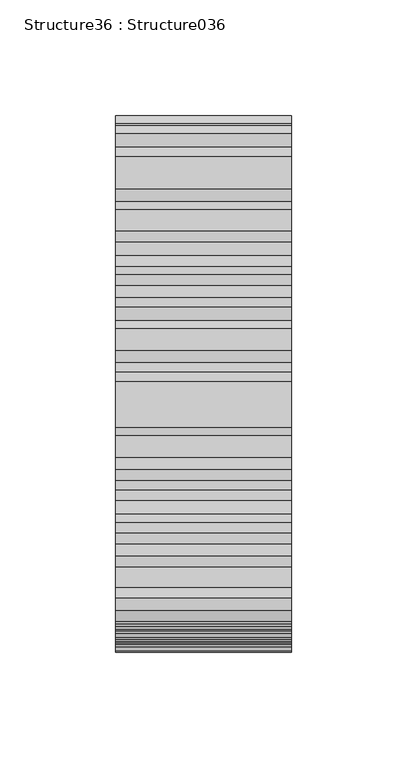
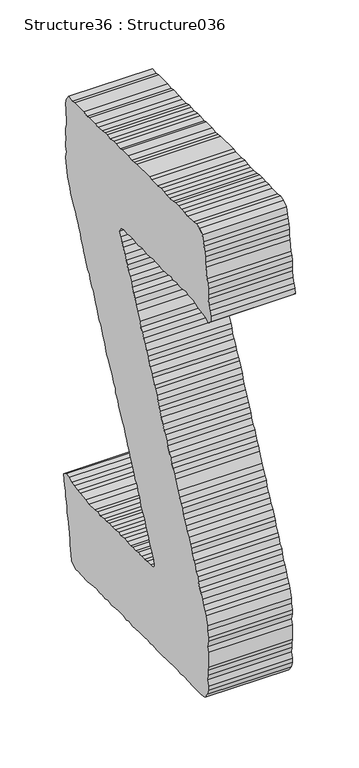
"""IFC4 building model written with IfcOpenShell, lengths in millimetres: proxy geometry, Structure36 : Structure036."""

from ifc_helpers import new_model, si_unit, frame, origin, place, context, project, spatial, polyline, outline, extrude, source, transform, mapped, element, save


def structure36_structure036_21f55036(model_context):
    return source(origin(), model_context, "Body", "SweptSolid", [
        extrude(outline(polyline([(252723.5287775, 3631.3410106), (252722.9447015, 3626.0554434), (252721.770131, 3621.3732075), (252720.5843283, 3616.69739), (252720.5843283, 3612.0135494), (252718.8353094, 3606.7295868), (252718.2512334, 3602.6298224), (252717.6607389, 3597.3538828), (252716.4845638, 3592.6700423), (252715.91172, 3589.1527492), (252714.7355449, 3584.4689087), (252714.1530735, 3579.7690221), (252713.5609744, 3573.9266571), (252713.5609744, 3569.8268927), (252712.3944269, 3565.1254015), (252711.8103509, 3561.025637), (252710.6341758, 3555.1848766), (252704.1932934, 3551.0658569), (252700.0839013, 3551.6675836), (252695.9841368, 3551.0658569), (252685.4418852, 3551.0658569), (252676.0661812, 3552.242032), (252671.9567891, 3552.242032), (252666.6904771, 3551.6675836), (252661.9970089, 3552.242032), (252658.4893435, 3551.0658569), (252653.79748, 3552.242032), (252647.947092, 3551.0658569), (252637.9792889, 3552.242032), (252629.1956838, 3552.242032), (252624.5022157, 3551.0658569), (252620.4024512, 3552.242032), (252615.1361393, 3551.0658569), (252609.8601997, 3551.0658569), (252605.1667315, 3551.6675836), (252596.3751035, 3551.6675836), (252591.1087915, 3552.242032), (252587.0090271, 3551.0658569), (252582.8996349, 3552.242032), (252577.0492469, 3551.0658569), (252572.3573834, 3551.6675836), (252567.0798392, 3551.0658569), (252562.3976033, 3551.6675836), (252544.811138, 3551.6675836), (252538.9623546, 3551.0658569), (252535.4450616, 3551.6675836), (252525.4756539, 3551.6675836), (252520.8030456, 3551.0658569), (252507.3179494, 3551.0658569), (252501.4579338, 3551.6675836), (252497.3581693, 3556.9258725), (252496.1835988, 3561.6257591), (252496.1835988, 3565.7094775), (252497.3581693, 3570.9854171), (252496.7756978, 3575.6853037), (252496.7756978, 3580.3691442), (252496.1835988, 3583.8864372), (252496.1835988, 3597.9540049), (252497.3581693, 3602.6298224), (252496.1835988, 3608.4705827), (252496.1835988, 3612.0135494), (252497.3581693, 3617.8559144), (252497.3581693, 3622.555801), (252499.7008918, 3630.7392839), (252501.4579338, 3634.2822506), (252503.8006563, 3638.3563415), (252505.5673259, 3643.0578326), (252507.3179494, 3648.3161216), (252509.668695, 3651.2589662), (252511.4177139, 3656.5429288), (252512.5922844, 3660.6250426), (252515.519083, 3663.5598643), (252517.2857525, 3669.4262983), (252518.4426723, 3672.3691429), (252521.9599654, 3677.0449604), (252522.5520645, 3681.7271964), (252524.310711, 3684.6443673), (252526.6534336, 3689.9540036), (252529.5770229, 3694.029699), (252531.3436925, 3698.1294635), (252533.678392, 3702.229228), (252536.0371606, 3706.3289925), (252536.6132137, 3711.6145597), (252538.9623546, 3714.5301261), (252541.2954496, 3719.2316172), (252543.6558228, 3723.9154578), (252547.7475643, 3732.7167134), (252549.5046062, 3736.7988273), (252551.2728803, 3740.9162424), (252553.6059753, 3743.8414364), (252554.7805458, 3749.117376), (252557.7041351, 3752.6170184), (252560.0468577, 3757.3185096), (252561.2230328, 3761.418274), (252563.5641508, 3765.5019925), (252565.3211927, 3769.0176809), (252567.0798392, 3773.7015215), (252570.0146608, 3778.4046172), (252571.7733074, 3783.0868532), (252573.5319539, 3786.6298199), (252574.6968968, 3791.3056374), (252577.0492469, 3795.4037973), (252579.3903649, 3800.0876378), (252580.5569124, 3803.0064134), (252584.0726008, 3807.714323), (252584.6663045, 3811.2043377), (252587.5931031, 3816.4883003), (252589.9326164, 3820.015221), (252591.1087915, 3824.1149855), (252592.8578104, 3828.2163546), (252595.7910275, 3833.4730389), (252597.549674, 3837.6000817), (252599.3083205, 3842.2758992), (252602.2431421, 3845.1914656), (252603.408085, 3850.4754282), (252607.5190817, 3857.5019912), (252609.8601997, 3862.2018778), (252611.0267471, 3867.4601667), (252613.3678651, 3871.5599312), (252616.2930591, 3875.0772243), (252616.8851582, 3879.7610648), (252619.2278807, 3883.8881076), (252622.1610977, 3887.9621984), (252622.7355461, 3892.6636896), (252625.0959194, 3895.5888836), (252626.8449383, 3900.2887701), (252629.7781553, 3904.9645876), (252631.5271742, 3909.0627475), (252633.8698967, 3912.5896682), (252636.2206423, 3916.6653636), (252633.2938437, 3921.3748778), (252628.6035848, 3922.5494483), (252623.3276452, 3921.3748778), (252618.6438047, 3922.5494483), (252614.5424356, 3922.5494483), (252609.8601997, 3921.3748778), (252605.7508076, 3921.3748778), (252600.4764726, 3922.5494483), (252596.9591795, 3921.9733953), (252592.283362, 3921.3748778), (252587.0090271, 3921.3748778), (252582.8996349, 3922.5494483), (252578.7982658, 3921.9733953), (252572.9398548, 3921.9733953), (252569.4305848, 3921.3748778), (252559.4627817, 3921.3748778), (252554.1964697, 3922.5494483), (252551.2728803, 3921.3748778), (252545.9889177, 3922.5494483), (252541.2954496, 3921.3748778), (252537.1940805, 3921.3748778), (252531.3436925, 3922.5494483), (252527.2375096, 3921.3748778), (252519.036376, 3921.3748778), (252513.185988, 3919.0321552), (252509.0765959, 3917.8479571), (252504.39436, 3917.2735087), (252500.2833633, 3916.6653636), (252495.5898951, 3914.3499193), (252491.4901306, 3917.8479571), (252492.0822297, 3922.5494483), (252493.8408762, 3926.6492128), (252495.0154467, 3931.3346579), (252495.5898951, 3937.1930689), (252496.1835988, 3940.718385), (252496.1835988, 3946.5511223), (252496.7756978, 3951.2606365), (252497.9502683, 3954.7506513), (252499.7008918, 3964.7361051), (252500.8738577, 3968.8198235), (252500.8738577, 3974.1214368), (252501.4579338, 3978.8036727), (252502.6325043, 3983.4794902), (252503.8006563, 3987.0048063), (252504.9752268, 3992.8375436), (252509.668695, 3996.390138), (252514.9350069, 3997.5486624), (252519.6188474, 3996.390138), (252528.4201031, 3996.390138), (252533.094316, 3997.5486624), (252538.3718602, 3996.9645864), (252543.0621191, 3997.5486624), (252547.7475643, 3997.5486624), (252551.2728803, 3996.9645864), (252557.1232683, 3996.390138), (252561.8135273, 3996.390138), (252565.9148964, 3996.9645864), (252570.5987369, 3997.5486624), (252575.8746765, 3996.9645864), (252585.2407529, 3996.9645864), (252588.766069, 3997.5486624), (252608.674397, 3997.5486624), (252612.7853937, 3996.9645864), (252616.8851582, 3996.390138), (252622.1610977, 3997.5486624), (252631.5271742, 3997.5486624), (252635.0460718, 3996.390138), (252640.9125059, 3997.5486624), (252645.0122704, 3997.5486624), (252650.2785823, 3996.9645864), (252654.9720505, 3997.5486624), (252658.4893435, 3997.5486624), (252663.1828117, 3996.390138), (252669.0331997, 3996.390138), (252673.7234586, 3996.9645864), (252683.0911396, 3996.9645864), (252686.6068281, 3996.390138), (252691.8827677, 3997.5486624), (252705.9423123, 3997.5486624), (252710.0436814, 3996.390138), (252715.91172, 3997.5486624), (252719.4290131, 3992.2614906), (252720.0130891, 3988.1633307), (252719.4290131, 3982.8793681), (252719.4290131, 3978.8036727), (252718.8353094, 3974.1214368), (252718.8353094, 3968.8198235), (252720.0130891, 3964.7361051), (252720.0130891, 3960.0602876), (252719.4290131, 3954.7506513), (252720.0130891, 3950.0940891), (252720.0130891, 3947.1496398), (252718.8353094, 3942.4770315), (252720.0130891, 3937.1930689), (252719.4290131, 3931.9058971), (252718.8353094, 3928.4158823), (252717.0766629, 3919.6066036), (252712.9672708, 3911.4054701), (252712.3944269, 3906.7328618), (252709.4596053, 3901.44569), (252707.7009588, 3897.9476522), (252704.7773694, 3893.822214), (252703.0187229, 3889.7208449), (252700.6776049, 3885.6210804), (252699.4998252, 3880.9452629), (252696.5762358, 3877.4456205), (252695.9841368, 3872.745734), (252693.0589428, 3867.4601667), (252691.8827677, 3863.9332461), (252689.5432543, 3859.2606378), (252687.7846078, 3855.7353217), (252685.4418852, 3850.4754282), (252682.5150866, 3847.5598618), (252681.9245922, 3843.432819), (252679.5738466, 3838.1761347), (252676.6486526, 3834.6588416), (252674.8980291, 3830.5574726), (252673.1313595, 3825.849563), (252670.7982646, 3821.1737455), (252667.85542, 3812.3901405), (252664.3397315, 3809.4729695), (252663.1828117, 3804.7730829), (252661.4145375, 3800.6717138), (252658.4893435, 3795.4037973), (252657.314773, 3791.8865042), (252655.5657541, 3787.2042683), (252652.6293279, 3783.0868532), (252651.456362, 3779.5872107), (252649.1040118, 3775.4874463), (252646.7628939, 3771.3860772), (252645.0122704, 3766.684586), (252642.0790533, 3762.5848215), (252641.4869543, 3758.485057), (252637.9792889, 3753.2171405), (252636.8111368, 3749.117376), (252634.4619958, 3744.9999608), (252632.1208778, 3740.3161203), (252630.3622313, 3736.2163558), (252628.0195088, 3732.7167134), (252626.2608622, 3727.4311462), (252623.9101166, 3723.3313817), (252622.7355461, 3720.4158154), (252620.9865272, 3716.2887726), (252618.6438047, 3710.4560353), (252615.7105877, 3706.3289925), (252611.6108232, 3698.1294635), (252611.0267471, 3694.6298211), (252607.5190817, 3689.9540036), (252606.3445112, 3685.8285655), (252603.408085, 3681.7271964), (252602.8256136, 3677.0449604), (252601.0605486, 3672.9435914), (252595.7910275, 3665.3265338), (252594.0323809, 3660.0682449), (252591.691263, 3655.3587307), (252589.342122, 3651.2589662), (252588.766069, 3647.1575971), (252585.2407529, 3642.4833842), (252583.491734, 3639.5405396), (252581.7250644, 3634.2822506), (252580.5569124, 3630.7392839), (252581.7250644, 3627.2396415), (252587.0090271, 3626.6571701), (252592.283362, 3627.2396415), (252596.3751035, 3626.6571701), (252601.0605486, 3626.6571701), (252606.3445112, 3627.2396415), (252610.4426711, 3626.0554434), (252615.1361393, 3626.6571701), (252618.6438047, 3626.0554434), (252623.9101166, 3626.6571701), (252628.0195088, 3627.2396415), (252633.8698967, 3626.0554434), (252637.3952128, 3627.2396415), (252642.6615248, 3626.6571701), (252647.3549929, 3626.6571701), (252652.0468565, 3627.2396415), (252656.7210694, 3626.0554434), (252660.2383624, 3626.6571701), (252666.1064011, 3626.0554434), (252670.2077702, 3627.2396415), (252674.8980291, 3626.0554434), (252684.2657101, 3626.0554434), (252688.9591783, 3627.2396415), (252697.7331557, 3628.4158166), (252701.2584717, 3628.998288), (252707.1168828, 3629.5984101), (252710.6341758, 3630.7392839), (252714.7355449, 3633.0980525), (252719.4290131, 3633.6821286), (252723.5287775, 3631.3410106)])), frame((-38594.2176606, 0.0, 0.0), z_axis=(1.0, 0.0, 0.0), x_axis=(0.0, 1.0, 0.0)), (0.0, 0.0, 1.0), 76.2),
    ])


if __name__ == "__main__":
    model = new_model("IFC4")
    model_context = context("Model", 3, world=origin())
    ifc_project = project(units=[si_unit("LENGTHUNIT", "METRE", prefix="MILLI")], contexts=[model_context])
    site = spatial("IfcSite", under=ifc_project)
    building = spatial("IfcBuilding", under=site)
    placement = place(None, origin())
    structure36_structure036_shape = structure36_structure036_21f55036(model_context)
    element("IfcBuildingElementProxy", 1, Name="Structure36 : Structure036", ObjectType="Structure36 : Structure036", at=placement, inside=building, context=model_context, shape_type="MappedRepresentation", body=[
        mapped(structure36_structure036_shape, transform((0.0, 0.0, 0.0), x_axis=(1.0, 0.0, 0.0), y_axis=(0.0, 1.0, 0.0), z_axis=(0.0, 0.0, 1.0))),
    ])
    save(model, "model.ifc")

# Revit data of these elements
# Type "Structure36 : Structure036"
#   NameOverride = "Structure036"
# Element 1 (IfcBuildingElementProxy, "Structure36 : Structure036")
#   Materials on its faces: "BRUSHED ALUM. LETTERING"
# Materials
#   "BRUSHED ALUM. LETTERING": class "Unassigned", colour RGB 169 181 186, transparency 0, Cost = 0
